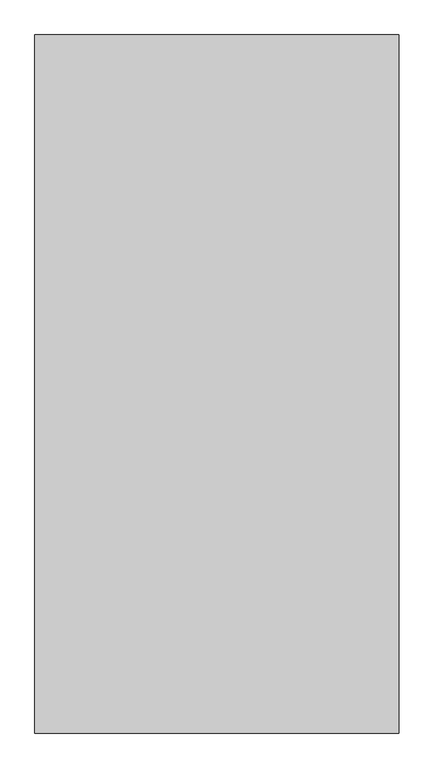
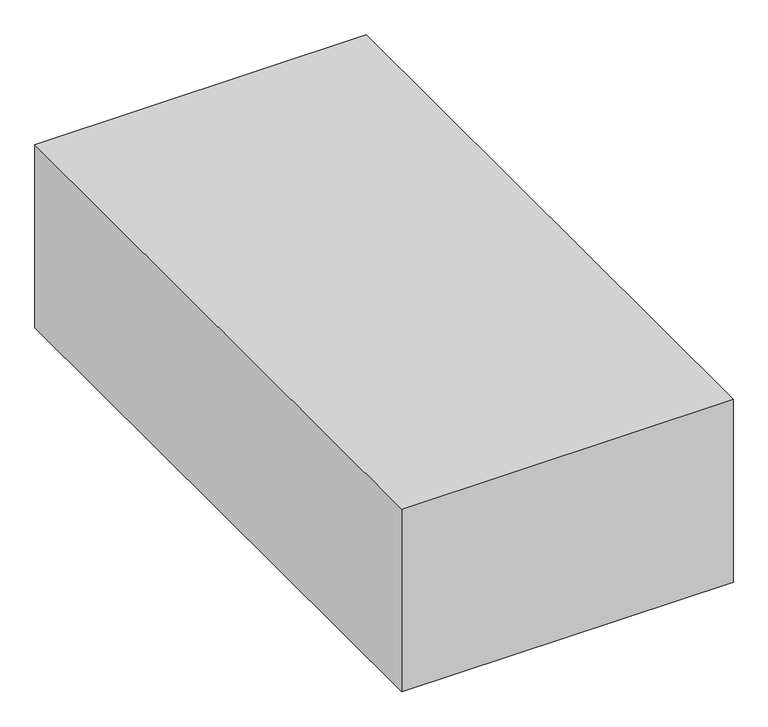
"""IFC4 building model written with IfcOpenShell, lengths in millimetres: proxy geometry, Space Planning Box_hec : Space Planning Box_hec."""

from ifc_helpers import new_model, si_unit, origin, origin_with_axes, place, context, project, spatial, polyline, outline, extrude, source, transform, mapped, element, save


def generic_models_ccc8c8c2(model_context):
    return source(origin(), model_context, "Body", "SweptSolid", [
        extrude(outline(polyline([(3000.0, 5750.0), (3000.0, -5750.0), (-3000.0, -5750.0), (-3000.0, 5750.0), (3000.0, 5750.0)])), origin_with_axes(), (0.0, 0.0, 1.0), 3500.0),
    ])


if __name__ == "__main__":
    model = new_model("IFC4")
    model_context = context("Model", 3, world=origin())
    ifc_project = project(units=[si_unit("LENGTHUNIT", "METRE", prefix="MILLI")], contexts=[model_context])
    site = spatial("IfcSite", under=ifc_project)
    building = spatial("IfcBuilding", under=site)
    placement = place(None, origin())
    generic_models_shape = generic_models_ccc8c8c2(model_context)
    element("IfcBuildingElementProxy", 1, Name="Space Planning Box_hec : Space Planning Box_hec", ObjectType="Space Planning Box_hec : Space Planning Box_hec", at=placement, inside=building, context=model_context, shape_type="MappedRepresentation", body=[
        mapped(generic_models_shape, transform((0.0, 0.0, 0.0), x_axis=(1.0, 0.0, 0.0), y_axis=(0.0, 1.0, 0.0), z_axis=(0.0, 0.0, 1.0))),
    ])
    save(model, "model.ifc")

# Revit data of these elements
# Type "Space Planning Box_hec : Space Planning Box_hec"
#   Type Comments = "..."
#   Room Name [instance default] = "?"
#   Interior Finish [instance default] = ""
#   Exterior Finish [instance default] = ""
#   Department [instance default] = ""
#   Assembly Code = "..."
#   ceiling height [instance default] = 0
#   Width [instance default] = 1524 mm
#   Program Area [instance default] = 0.00 m²
#   Length [instance default] = 1524 mm
#   Height [instance default] = 1524 mm
#   Area [instance default] = 2.32258 m²
#   Fill Color [instance default] = Cyan
#   Default Elevation = 0
# Element 1 (IfcBuildingElementProxy, "Space Planning Box_hec : Space Planning Box_hec")
#   Room Name = "Meeting Room-1"
#   Exterior Finish = "RF1..N/A,,EW1..EW2..N/A"
#   Department = "AR"
#   Width = 6000 mm
#   Program Area = 69.00 m²
#   Length = 11500 mm
#   Height = 3500 mm
#   Area = 69.00 m²
#   Materials on its faces: "Cyan"
# Materials
#   "Cyan": class "Generic", colour RGB 0 255 255, transparency 0.2, Cost = 0
